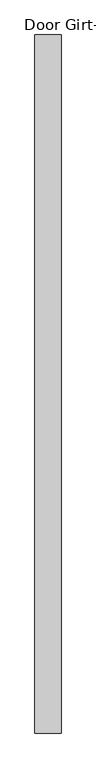
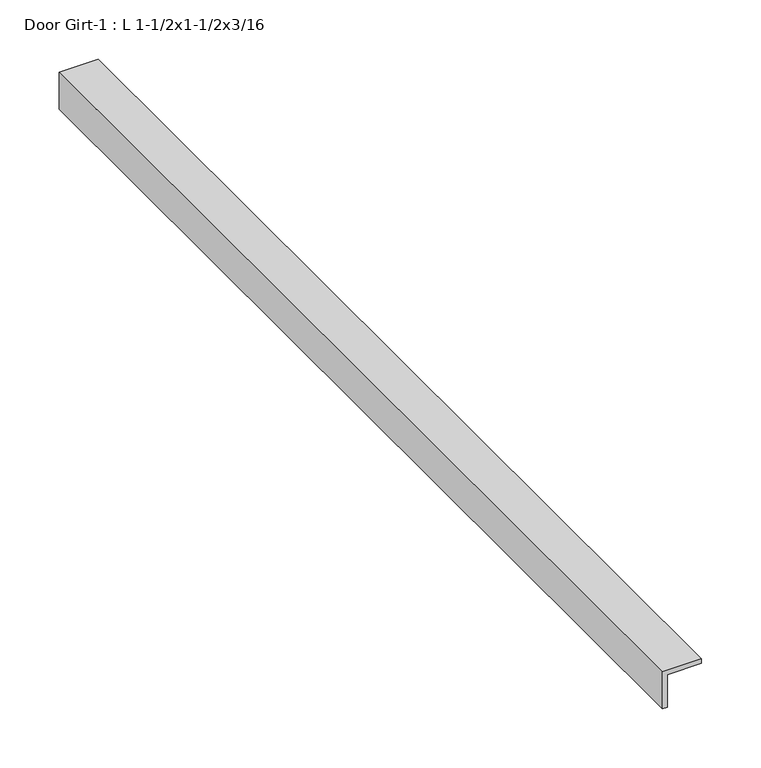
"""IFC4 building model written with IfcOpenShell, lengths in millimetres: proxy geometry, Door Girt-1 : L 1-1/2x1-1/2x3/16."""

import ifcopenshell
import ifcopenshell.guid

model = None  # the IFC model being written
_history = None  # IfcOwnerHistory: only IFC2X3 demands one
_inside = {}  # id of a spatial element -> (the spatial element, [elements in it])
_under = {}  # id of a project, library or spatial element -> (it, [spatial elements below it])
_declared = {}  # id of a project -> (the project, [libraries it declares])
_typed = {}  # id of a type object -> (the type object, [elements of that type])
_made_of = {}  # id of a material, layer set ... -> (it, [elements and type objects made of it])


def new_model(schema):
    """Start an empty IFC model of exactly this schema.

    Asked for "IFC4X3", IfcOpenShell would pick the latest addendum, in which some entities
    have other attributes; the version numbers below select the first issue.
    IFC2X3 requires an IfcOwnerHistory on every rooted entity: one is made here for all.
    """
    global model, _history
    if schema == "IFC4X3":
        model = ifcopenshell.file(schema_version=(4, 3, 0, 0))
    else:
        model = ifcopenshell.file(schema=schema)
    _inside.clear()
    _under.clear()
    _declared.clear()
    _typed.clear()
    _made_of.clear()
    _history = None
    if model.schema == "IFC2X3":
        org = make("IfcOrganization", Name="unknown")
        user = make(
            "IfcPersonAndOrganization",
            ThePerson=make("IfcPerson", FamilyName="unknown"),
            TheOrganization=org,
        )
        app = make(
            "IfcApplication",
            ApplicationDeveloper=org,
            Version="unknown",
            ApplicationFullName="unknown",
            ApplicationIdentifier="unknown",
        )
        _history = make(
            "IfcOwnerHistory",
            OwningUser=user,
            OwningApplication=app,
            ChangeAction="ADDED",
            CreationDate=0,
        )
    return model


def make(cls, **values):
    """One entity of the class cls with the attributes given. An attribute that is None is left unset."""
    return model.create_entity(
        cls, **{name: value for name, value in values.items() if value is not None}
    )


def rooted(cls, **values):
    """An entity with a GlobalId (a new one), such as an element, a storey or a relation."""
    return make(cls, GlobalId=ifcopenshell.guid.new(), OwnerHistory=_history, **values)


def si_unit(unit_type, name, prefix=None):
    """IfcSIUnit, for example si_unit("LENGTHUNIT", "METRE", prefix="MILLI")."""
    return make("IfcSIUnit", UnitType=unit_type, Prefix=prefix, Name=name)


def assignment(units):
    """IfcUnitAssignment: the units of a project."""
    return None if units is None else make("IfcUnitAssignment", Units=units)


def point(xyz):
    """IfcCartesianPoint."""
    return None if xyz is None else make("IfcCartesianPoint", Coordinates=xyz)


def direction(xyz):
    """IfcDirection."""
    return None if xyz is None else make("IfcDirection", DirectionRatios=xyz)


def frame(location, z_axis=None, x_axis=None):
    """IfcAxis2Placement3D, a coordinate frame: its origin and axes. An axis left out is left unset."""
    return make(
        "IfcAxis2Placement3D",
        Location=point(location),
        Axis=direction(z_axis),
        RefDirection=direction(x_axis),
    )


def origin():
    """The frame at (0, 0, 0) with its axes left unset."""
    return frame((0.0, 0.0, 0.0))


def place(relative_to, where):
    """IfcLocalPlacement: puts the frame where relative to a parent placement (None: the world)."""
    return make(
        "IfcLocalPlacement", PlacementRelTo=relative_to, RelativePlacement=where
    )


def context(
    kind, dimensions, precision=None, world=None, true_north=None, identifier=None
):
    """IfcGeometricRepresentationContext, for example the 3D "Model" context."""
    return make(
        "IfcGeometricRepresentationContext",
        ContextIdentifier=identifier,
        ContextType=kind,
        CoordinateSpaceDimension=dimensions,
        Precision=precision,
        WorldCoordinateSystem=world,
        TrueNorth=true_north,
    )


def project(units=None, contexts=None):
    """IfcProject with its units and contexts."""
    return rooted(
        "IfcProject",
        Name="project",
        RepresentationContexts=contexts,
        UnitsInContext=assignment(units),
    )


def spatial(cls, under=None, at=None, **own):
    """A site, building, storey or space (cls), placed at a placement, below another one or the project."""
    s = rooted(cls, ObjectPlacement=at, **own)
    if under is not None:
        _under.setdefault(under.id(), (under, []))[1].append(s)
    return s


def polyline(points):
    """IfcPolyline through the points."""
    return make("IfcPolyline", Points=[point(p) for p in points])


def outline(outer, holes=None, kind="AREA"):
    """IfcArbitraryClosedProfileDef: a profile drawn as a closed curve; with holes, ...WithVoids."""
    if holes is None:
        return make("IfcArbitraryClosedProfileDef", ProfileType=kind, OuterCurve=outer)
    return make(
        "IfcArbitraryProfileDefWithVoids",
        ProfileType=kind,
        OuterCurve=outer,
        InnerCurves=holes,
    )


def extrude(swept, where, along, depth):
    """IfcExtrudedAreaSolid: the profile swept, set in the frame where, extruded along a direction by depth."""
    return make(
        "IfcExtrudedAreaSolid",
        SweptArea=swept,
        Position=where,
        ExtrudedDirection=direction(along),
        Depth=depth,
    )


def shape(context_of_items, identifier, shape_type, items):
    """IfcShapeRepresentation: the items that make up one representation, for example the "Body"."""
    return make(
        "IfcShapeRepresentation",
        ContextOfItems=context_of_items,
        RepresentationIdentifier=identifier,
        RepresentationType=shape_type,
        Items=items,
    )


def source(mapping_origin, context_of_items, identifier, shape_type, items):
    """IfcRepresentationMap: a shape defined once, which mapped items show again and again."""
    return make(
        "IfcRepresentationMap",
        MappingOrigin=mapping_origin,
        MappedRepresentation=shape(context_of_items, identifier, shape_type, items),
    )


def transform(
    local_origin,
    x_axis=None,
    y_axis=None,
    z_axis=None,
    scale=None,
    scale2=None,
    scale3=None,
    uniform=True,
):
    """IfcCartesianTransformationOperator3D, or its non-uniform kind. x_axis, y_axis, z_axis: its Axis1, 2, 3."""
    if uniform:
        return make(
            "IfcCartesianTransformationOperator3D",
            Axis1=direction(x_axis),
            Axis2=direction(y_axis),
            LocalOrigin=point(local_origin),
            Scale=scale,
            Axis3=direction(z_axis),
        )
    return make(
        "IfcCartesianTransformationOperator3DnonUniform",
        Axis1=direction(x_axis),
        Axis2=direction(y_axis),
        LocalOrigin=point(local_origin),
        Scale=scale,
        Axis3=direction(z_axis),
        Scale2=scale2,
        Scale3=scale3,
    )


def mapped(mapping_source, mapping_target):
    """IfcMappedItem: shows the shape of a source again, moved by a transform."""
    return make(
        "IfcMappedItem", MappingSource=mapping_source, MappingTarget=mapping_target
    )


def made_of(thing, what):
    """Note that an element or type object is made of a material, layer set ...; save() writes the relation."""
    if what is not None:
        _made_of.setdefault(what.id(), (what, []))[1].append(thing)
    return thing


def element(
    cls,
    number,
    at=None,
    inside=None,
    cuts=None,
    type_object=None,
    material=None,
    context=None,
    identifier="Body",
    shape_type=None,
    held_by="IfcProductDefinitionShape",
    body=None,
    shapes=None,
    **own,
):
    """One element of the class cls, such as IfcWall. Its Tag is "e" and its number.

    at: its placement. inside: the storey or other place that contains it. cuts: it is an
    opening in that element (IfcRelVoidsElement). A single representation is given by context,
    identifier, shape_type and body (its items); several are given by shapes. held_by: the class
    of the entity that holds the representations. save() writes the other relations.
    """
    e = rooted(cls, Tag="e%d" % number, ObjectPlacement=at, **own)
    if body is not None:
        shapes = [shape(context, identifier, shape_type, body)]
    if shapes is not None:
        e.Representation = make(held_by, Representations=shapes)
    if inside is not None:
        _inside.setdefault(inside.id(), (inside, []))[1].append(e)
    if cuts is not None:
        rooted(
            "IfcRelVoidsElement", RelatingBuildingElement=cuts, RelatedOpeningElement=e
        )
    if type_object is not None:
        _typed.setdefault(type_object.id(), (type_object, []))[1].append(e)
    return made_of(e, material)


def aggregate(whole, parts):
    """IfcRelAggregates: a whole, such as a stair, and the parts it consists of."""
    return rooted("IfcRelAggregates", RelatingObject=whole, RelatedObjects=parts)


def save(model, path):
    """Write the relations noted so far, then the file.

    IfcRelAggregates (storeys below a building ...), IfcRelContainedInSpatialStructure (elements
    in a storey), IfcRelDefinesByType, IfcRelAssociatesMaterial and IfcRelDeclares: one each for
    every whole, place, type object, material and project.
    """
    for whole, parts in _under.values():
        aggregate(whole, parts)
    for where, things in _inside.values():
        rooted(
            "IfcRelContainedInSpatialStructure",
            RelatedElements=things,
            RelatingStructure=where,
        )
    for kind, things in _typed.values():
        rooted("IfcRelDefinesByType", RelatedObjects=things, RelatingType=kind)
    for what, things in _made_of.values():
        rooted("IfcRelAssociatesMaterial", RelatedObjects=things, RelatingMaterial=what)
    for by, libraries in _declared.values():
        rooted("IfcRelDeclares", RelatingContext=by, RelatedDefinitions=libraries)
    model.write(path)


def door_girt_1_l_1_1_2x1_1_2x3_16_e85b96be(model_context):
    return source(origin(), model_context, "Body", "SweptSolid", [
        extrude(outline(polyline([(1625.6, 587403.9934739), (1625.6, 587365.8934739), (1587.5, 587365.8934739), (1587.5, 587370.6559739), (1620.8375, 587370.6559739), (1620.8375, 587403.9934739), (1625.6, 587403.9934739)])), frame((0.0, -532839.3663841, 0.0), z_axis=(0.0, 1.0, 0.0), x_axis=(0.0, 0.0, 1.0)), (0.0, 0.0, 1.0), 1017.5875),
    ])


if __name__ == "__main__":
    model = new_model("IFC4")
    model_context = context("Model", 3, world=origin())
    ifc_project = project(units=[si_unit("LENGTHUNIT", "METRE", prefix="MILLI")], contexts=[model_context])
    site = spatial("IfcSite", under=ifc_project)
    building = spatial("IfcBuilding", under=site)
    placement = place(None, origin())
    door_girt_1_l_1_1_2x1_1_2x3_16_shape = door_girt_1_l_1_1_2x1_1_2x3_16_e85b96be(model_context)
    element("IfcBuildingElementProxy", 1, Name="Door Girt-1 : L 1-1/2x1-1/2x3/16", ObjectType="Door Girt-1 : L 1-1/2x1-1/2x3/16", at=placement, inside=building, context=model_context, shape_type="MappedRepresentation", body=[
        mapped(door_girt_1_l_1_1_2x1_1_2x3_16_shape, transform((0.0, 0.0, 0.0), x_axis=(1.0, 0.0, 0.0), y_axis=(0.0, 1.0, 0.0), z_axis=(0.0, 0.0, 1.0))),
    ])
    save(model, "model.ifc")

# Revit data of these elements
# Element 1 (IfcBuildingElementProxy, "Door Girt-1 : L 1-1/2x1-1/2x3/16")
#   Materials on its faces: "1-1/2\"X1-1/2\" GALV. STL L"
# Materials
#   "1-1/2\"X1-1/2\" GALV. STL L": class "Generic", colour RGB 211 211 207, transparency 0, Cost = 0
